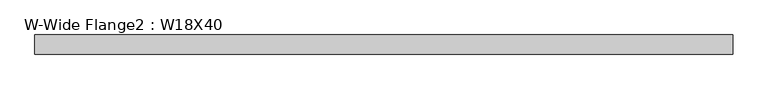
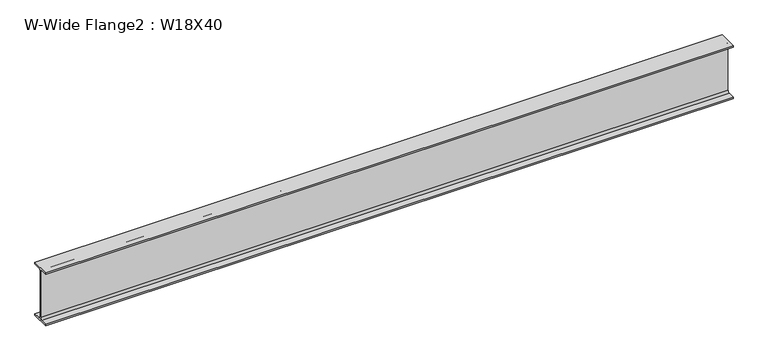
"""IFC4 building model written with IfcOpenShell, lengths in millimetres: beam geometry, W-Wide Flange2 : W18X40."""

import ifcopenshell
import ifcopenshell.guid

model = None  # the IFC model being written
_history = None  # IfcOwnerHistory: only IFC2X3 demands one
_inside = {}  # id of a spatial element -> (the spatial element, [elements in it])
_under = {}  # id of a project, library or spatial element -> (it, [spatial elements below it])
_declared = {}  # id of a project -> (the project, [libraries it declares])
_typed = {}  # id of a type object -> (the type object, [elements of that type])
_made_of = {}  # id of a material, layer set ... -> (it, [elements and type objects made of it])


def new_model(schema):
    """Start an empty IFC model of exactly this schema.

    Asked for "IFC4X3", IfcOpenShell would pick the latest addendum, in which some entities
    have other attributes; the version numbers below select the first issue.
    IFC2X3 requires an IfcOwnerHistory on every rooted entity: one is made here for all.
    """
    global model, _history
    if schema == "IFC4X3":
        model = ifcopenshell.file(schema_version=(4, 3, 0, 0))
    else:
        model = ifcopenshell.file(schema=schema)
    _inside.clear()
    _under.clear()
    _declared.clear()
    _typed.clear()
    _made_of.clear()
    _history = None
    if model.schema == "IFC2X3":
        org = make("IfcOrganization", Name="unknown")
        user = make(
            "IfcPersonAndOrganization",
            ThePerson=make("IfcPerson", FamilyName="unknown"),
            TheOrganization=org,
        )
        app = make(
            "IfcApplication",
            ApplicationDeveloper=org,
            Version="unknown",
            ApplicationFullName="unknown",
            ApplicationIdentifier="unknown",
        )
        _history = make(
            "IfcOwnerHistory",
            OwningUser=user,
            OwningApplication=app,
            ChangeAction="ADDED",
            CreationDate=0,
        )
    return model


def make(cls, **values):
    """One entity of the class cls with the attributes given. An attribute that is None is left unset."""
    return model.create_entity(
        cls, **{name: value for name, value in values.items() if value is not None}
    )


def rooted(cls, **values):
    """An entity with a GlobalId (a new one), such as an element, a storey or a relation."""
    return make(cls, GlobalId=ifcopenshell.guid.new(), OwnerHistory=_history, **values)


def si_unit(unit_type, name, prefix=None):
    """IfcSIUnit, for example si_unit("LENGTHUNIT", "METRE", prefix="MILLI")."""
    return make("IfcSIUnit", UnitType=unit_type, Prefix=prefix, Name=name)


def assignment(units):
    """IfcUnitAssignment: the units of a project."""
    return None if units is None else make("IfcUnitAssignment", Units=units)


def point(xyz):
    """IfcCartesianPoint."""
    return None if xyz is None else make("IfcCartesianPoint", Coordinates=xyz)


def direction(xyz):
    """IfcDirection."""
    return None if xyz is None else make("IfcDirection", DirectionRatios=xyz)


def frame(location, z_axis=None, x_axis=None):
    """IfcAxis2Placement3D, a coordinate frame: its origin and axes. An axis left out is left unset."""
    return make(
        "IfcAxis2Placement3D",
        Location=point(location),
        Axis=direction(z_axis),
        RefDirection=direction(x_axis),
    )


def frame_2d(location, x_axis=None):
    """IfcAxis2Placement2D, a coordinate frame in the plane: its origin and x axis."""
    return make(
        "IfcAxis2Placement2D", Location=point(location), RefDirection=direction(x_axis)
    )


def origin():
    """The frame at (0, 0, 0) with its axes left unset."""
    return frame((0.0, 0.0, 0.0))


def place(relative_to, where):
    """IfcLocalPlacement: puts the frame where relative to a parent placement (None: the world)."""
    return make(
        "IfcLocalPlacement", PlacementRelTo=relative_to, RelativePlacement=where
    )


def context(
    kind, dimensions, precision=None, world=None, true_north=None, identifier=None
):
    """IfcGeometricRepresentationContext, for example the 3D "Model" context."""
    return make(
        "IfcGeometricRepresentationContext",
        ContextIdentifier=identifier,
        ContextType=kind,
        CoordinateSpaceDimension=dimensions,
        Precision=precision,
        WorldCoordinateSystem=world,
        TrueNorth=true_north,
    )


def project(units=None, contexts=None):
    """IfcProject with its units and contexts."""
    return rooted(
        "IfcProject",
        Name="project",
        RepresentationContexts=contexts,
        UnitsInContext=assignment(units),
    )


def spatial(cls, under=None, at=None, **own):
    """A site, building, storey or space (cls), placed at a placement, below another one or the project."""
    s = rooted(cls, ObjectPlacement=at, **own)
    if under is not None:
        _under.setdefault(under.id(), (under, []))[1].append(s)
    return s


def polyline(points):
    """IfcPolyline through the points."""
    return make("IfcPolyline", Points=[point(p) for p in points])


def circle_curve(where, radius):
    """IfcCircle in the frame where."""
    return make("IfcCircle", Position=where, Radius=radius)


def trimmed(basis, trim1, trim2, sense, master):
    """IfcTrimmedCurve: the piece of a basis curve between two trims."""
    return make(
        "IfcTrimmedCurve",
        BasisCurve=basis,
        Trim1=trim1,
        Trim2=trim2,
        SenseAgreement=sense,
        MasterRepresentation=master,
    )


def segment(curve, same_sense, transition):
    """IfcCompositeCurveSegment."""
    return make(
        "IfcCompositeCurveSegment",
        Transition=transition,
        SameSense=same_sense,
        ParentCurve=curve,
    )


def composite_curve(segments, self_intersect=None):
    """IfcCompositeCurve: segments joined end to end."""
    return make("IfcCompositeCurve", Segments=segments, SelfIntersect=self_intersect)


def outline(outer, holes=None, kind="AREA"):
    """IfcArbitraryClosedProfileDef: a profile drawn as a closed curve; with holes, ...WithVoids."""
    if holes is None:
        return make("IfcArbitraryClosedProfileDef", ProfileType=kind, OuterCurve=outer)
    return make(
        "IfcArbitraryProfileDefWithVoids",
        ProfileType=kind,
        OuterCurve=outer,
        InnerCurves=holes,
    )


def extrude(swept, where, along, depth):
    """IfcExtrudedAreaSolid: the profile swept, set in the frame where, extruded along a direction by depth."""
    return make(
        "IfcExtrudedAreaSolid",
        SweptArea=swept,
        Position=where,
        ExtrudedDirection=direction(along),
        Depth=depth,
    )


def shape(context_of_items, identifier, shape_type, items):
    """IfcShapeRepresentation: the items that make up one representation, for example the "Body"."""
    return make(
        "IfcShapeRepresentation",
        ContextOfItems=context_of_items,
        RepresentationIdentifier=identifier,
        RepresentationType=shape_type,
        Items=items,
    )


def source(mapping_origin, context_of_items, identifier, shape_type, items):
    """IfcRepresentationMap: a shape defined once, which mapped items show again and again."""
    return make(
        "IfcRepresentationMap",
        MappingOrigin=mapping_origin,
        MappedRepresentation=shape(context_of_items, identifier, shape_type, items),
    )


def transform(
    local_origin,
    x_axis=None,
    y_axis=None,
    z_axis=None,
    scale=None,
    scale2=None,
    scale3=None,
    uniform=True,
):
    """IfcCartesianTransformationOperator3D, or its non-uniform kind. x_axis, y_axis, z_axis: its Axis1, 2, 3."""
    if uniform:
        return make(
            "IfcCartesianTransformationOperator3D",
            Axis1=direction(x_axis),
            Axis2=direction(y_axis),
            LocalOrigin=point(local_origin),
            Scale=scale,
            Axis3=direction(z_axis),
        )
    return make(
        "IfcCartesianTransformationOperator3DnonUniform",
        Axis1=direction(x_axis),
        Axis2=direction(y_axis),
        LocalOrigin=point(local_origin),
        Scale=scale,
        Axis3=direction(z_axis),
        Scale2=scale2,
        Scale3=scale3,
    )


def mapped(mapping_source, mapping_target):
    """IfcMappedItem: shows the shape of a source again, moved by a transform."""
    return make(
        "IfcMappedItem", MappingSource=mapping_source, MappingTarget=mapping_target
    )


def made_of(thing, what):
    """Note that an element or type object is made of a material, layer set ...; save() writes the relation."""
    if what is not None:
        _made_of.setdefault(what.id(), (what, []))[1].append(thing)
    return thing


def element(
    cls,
    number,
    at=None,
    inside=None,
    cuts=None,
    type_object=None,
    material=None,
    context=None,
    identifier="Body",
    shape_type=None,
    held_by="IfcProductDefinitionShape",
    body=None,
    shapes=None,
    **own,
):
    """One element of the class cls, such as IfcWall. Its Tag is "e" and its number.

    at: its placement. inside: the storey or other place that contains it. cuts: it is an
    opening in that element (IfcRelVoidsElement). A single representation is given by context,
    identifier, shape_type and body (its items); several are given by shapes. held_by: the class
    of the entity that holds the representations. save() writes the other relations.
    """
    e = rooted(cls, Tag="e%d" % number, ObjectPlacement=at, **own)
    if body is not None:
        shapes = [shape(context, identifier, shape_type, body)]
    if shapes is not None:
        e.Representation = make(held_by, Representations=shapes)
    if inside is not None:
        _inside.setdefault(inside.id(), (inside, []))[1].append(e)
    if cuts is not None:
        rooted(
            "IfcRelVoidsElement", RelatingBuildingElement=cuts, RelatedOpeningElement=e
        )
    if type_object is not None:
        _typed.setdefault(type_object.id(), (type_object, []))[1].append(e)
    return made_of(e, material)


def aggregate(whole, parts):
    """IfcRelAggregates: a whole, such as a stair, and the parts it consists of."""
    return rooted("IfcRelAggregates", RelatingObject=whole, RelatedObjects=parts)


def save(model, path):
    """Write the relations noted so far, then the file.

    IfcRelAggregates (storeys below a building ...), IfcRelContainedInSpatialStructure (elements
    in a storey), IfcRelDefinesByType, IfcRelAssociatesMaterial and IfcRelDeclares: one each for
    every whole, place, type object, material and project.
    """
    for whole, parts in _under.values():
        aggregate(whole, parts)
    for where, things in _inside.values():
        rooted(
            "IfcRelContainedInSpatialStructure",
            RelatedElements=things,
            RelatingStructure=where,
        )
    for kind, things in _typed.values():
        rooted("IfcRelDefinesByType", RelatedObjects=things, RelatingType=kind)
    for what, things in _made_of.values():
        rooted("IfcRelAssociatesMaterial", RelatedObjects=things, RelatingMaterial=what)
    for by, libraries in _declared.values():
        rooted("IfcRelDeclares", RelatingContext=by, RelatedDefinitions=libraries)
    model.write(path)


def w_wide_flange2_w18x40_42c25f9a(model_context):
    return source(origin(), model_context, "Body", "SweptSolid", [
        extrude(outline(composite_curve([segment(polyline([(76.454, -213.995), (76.454, -227.33), (-76.454, -227.33), (-76.454, -213.995), (-20.828, -213.995)]), True, "CONTINUOUS"), segment(trimmed(circle_curve(frame_2d((-20.828, -197.1675)), 16.8275), [point((-20.828, -213.995))], [point((-4.0005, -197.1675))], True, "CARTESIAN"), True, "CONTINUOUS"), segment(polyline([(-4.0005, -197.1675), (-4.0005, 197.1675)]), True, "CONTINUOUS"), segment(trimmed(circle_curve(frame_2d((-20.828, 197.1675)), 16.8275), [point((-4.0005, 197.1675))], [point((-20.828, 213.995))], True, "CARTESIAN"), True, "CONTINUOUS"), segment(polyline([(-20.828, 213.995), (-76.454, 213.995), (-76.454, 227.33), (76.454, 227.33), (76.454, 213.995), (20.828, 213.995)]), True, "CONTINUOUS"), segment(trimmed(circle_curve(frame_2d((20.828, 197.1675)), 16.8275), [point((20.828, 213.995))], [point((4.0005, 197.1675))], True, "CARTESIAN"), True, "CONTINUOUS"), segment(polyline([(4.0005, 197.1675), (4.0005, -197.1675)]), True, "CONTINUOUS"), segment(trimmed(circle_curve(frame_2d((20.828, -197.1675)), 16.8275), [point((4.0005, -197.1675))], [point((20.828, -213.995))], True, "CARTESIAN"), True, "CONTINUOUS"), segment(polyline([(20.828, -213.995), (76.454, -213.995)]), True, "CONTINUOUS")], self_intersect=False)), frame((-2756.69375, 0.0, 0.0), z_axis=(1.0, 0.0, 0.0), x_axis=(0.0, 1.0, 0.0)), (0.0, 0.0, 1.0), 5570.5375),
    ])


if __name__ == "__main__":
    model = new_model("IFC4")
    model_context = context("Model", 3, world=origin())
    ifc_project = project(units=[si_unit("LENGTHUNIT", "METRE", prefix="MILLI")], contexts=[model_context])
    site = spatial("IfcSite", under=ifc_project)
    building = spatial("IfcBuilding", under=site)
    placement = place(None, origin())
    w_wide_flange2_w18x40_shape = w_wide_flange2_w18x40_42c25f9a(model_context)
    element("IfcBeam", 1, ObjectType="W-Wide Flange2 : W18X40", at=placement, inside=building, context=model_context, shape_type="MappedRepresentation", body=[
        mapped(w_wide_flange2_w18x40_shape, transform((0.0, 0.0, 0.0), x_axis=(1.0, 0.0, 0.0), y_axis=(0.0, 1.0, 0.0), z_axis=(0.0, 0.0, 1.0))),
    ])
    save(model, "model.ifc")

# Revit data of these elements
# Type "W-Wide Flange2 : W18X40"
#   Assembly Code = "B10"
#   W = 40
#   Length [instance default] = 5' - 0"
#   bf = 0' - 6.02"
#   d = 1' - 5.9"
#   k = 0' - 1 3/16"
#   k2 = 0' - 0.6625"
#   tf = 0' - 0.525"
#   tw = 0' - 0.315"
#   A = 0.0819444 SF
#   Structural Material [instance default] = Steel ASTM A992
# Element 1 (IfcBeam, "W-Wide Flange2 : W18X40")
#   Materials on its faces: "Steel ASTM A992"
# Materials
#   "Steel ASTM A992": class "Metal", colour RGB 199 199 199, transparency 0, Description = "Structural steel 50ksi", Cost = 0
